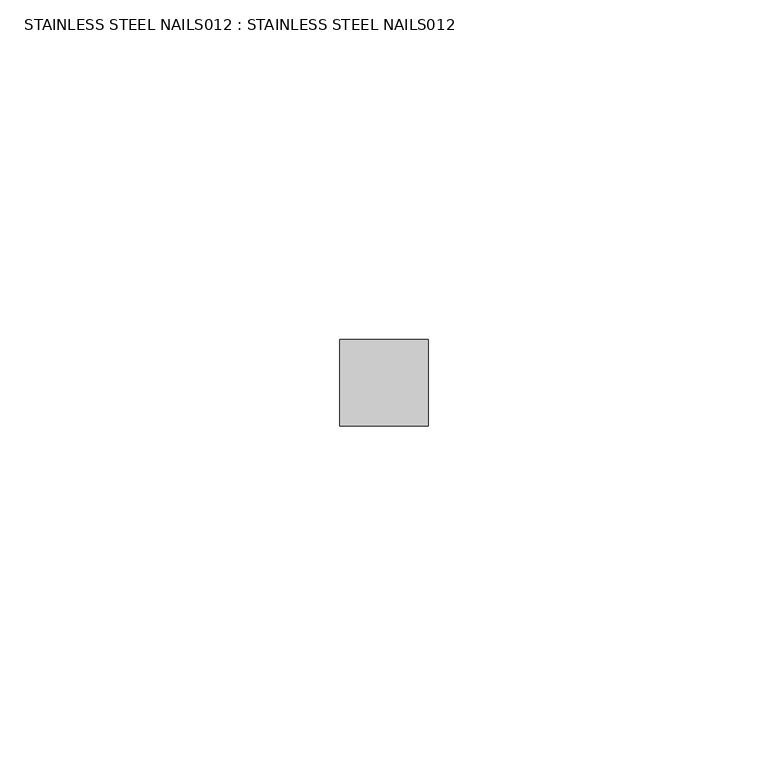
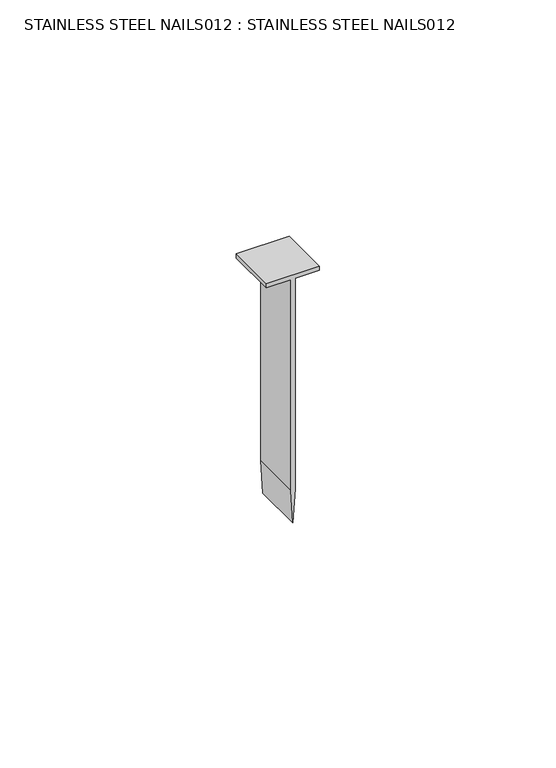
"""IFC4 building model written with IfcOpenShell, lengths in millimetres: proxy geometry, STAINLESS STEEL NAILS012 : STAINLESS STEEL NAILS012."""

from ifc_helpers import new_model, si_unit, frame, origin, place, context, project, spatial, polyline, outline, extrude, source, transform, mapped, element, save


def stainless_steel_nails012_stainless_steel_nails012_1b529cbc(model_context):
    return source(origin(), model_context, "Body", "SweptSolid", [
        extrude(outline(polyline([(40259.5998489, -4949.0239115), (40259.5998489, -4943.0663189), (40205.2737053, -4943.0663189), (40196.608116, -4942.5247196), (40205.2737053, -4941.9831203), (40259.5998489, -4941.9831203), (40259.5998489, -4936.0255277), (40260.6830476, -4936.0255277), (40260.6830476, -4949.0239115), (40259.5998489, -4949.0239115)])), frame((0.0, -1065.5906573, 0.0), z_axis=(0.0, 1.0, 0.0), x_axis=(0.0, 0.0, 1.0)), (0.0, 0.0, 1.0), 12.7),
    ])


if __name__ == "__main__":
    model = new_model("IFC4")
    model_context = context("Model", 3, world=origin())
    ifc_project = project(units=[si_unit("LENGTHUNIT", "METRE", prefix="MILLI")], contexts=[model_context])
    site = spatial("IfcSite", under=ifc_project)
    building = spatial("IfcBuilding", under=site)
    placement = place(None, origin())
    stainless_steel_nails012_stainless_steel_nails012_shape = stainless_steel_nails012_stainless_steel_nails012_1b529cbc(model_context)
    element("IfcBuildingElementProxy", 1, Name="STAINLESS STEEL NAILS012 : STAINLESS STEEL NAILS012", ObjectType="STAINLESS STEEL NAILS012 : STAINLESS STEEL NAILS012", at=placement, inside=building, context=model_context, shape_type="MappedRepresentation", body=[
        mapped(stainless_steel_nails012_stainless_steel_nails012_shape, transform((0.0, 0.0, 0.0), x_axis=(1.0, 0.0, 0.0), y_axis=(0.0, 1.0, 0.0), z_axis=(0.0, 0.0, 1.0))),
    ])
    save(model, "model.ifc")

# Revit data of these elements
# Type "STAINLESS STEEL NAILS012 : STAINLESS STEEL NAILS012"
#   NameOverride = "STAINLESS STEEL NAILS012"
# Element 1 (IfcBuildingElementProxy, "STAINLESS STEEL NAILS012 : STAINLESS STEEL NAILS012")
#   Materials on its faces: "1 3/4\" STAINLESS STEEL RINGSHANK 5D COMMON NAILS @ 4\" (101.6MM) O.C. FIRESTONE PROVIDED MAX., 1/2\" STAGGERED"
# Materials
#   "1 3/4\" STAINLESS STEEL RINGSHANK 5D COMMON NAILS @ 4\" (101.6MM) O.C. FIRESTONE PROVIDED MAX., 1/2\" STAGGERED": class "Unassigned", colour RGB 255 255 255, transparency 0
